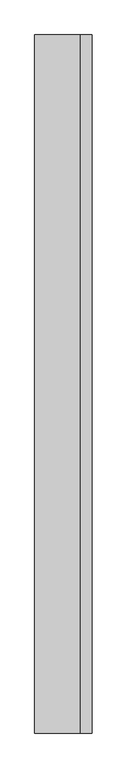
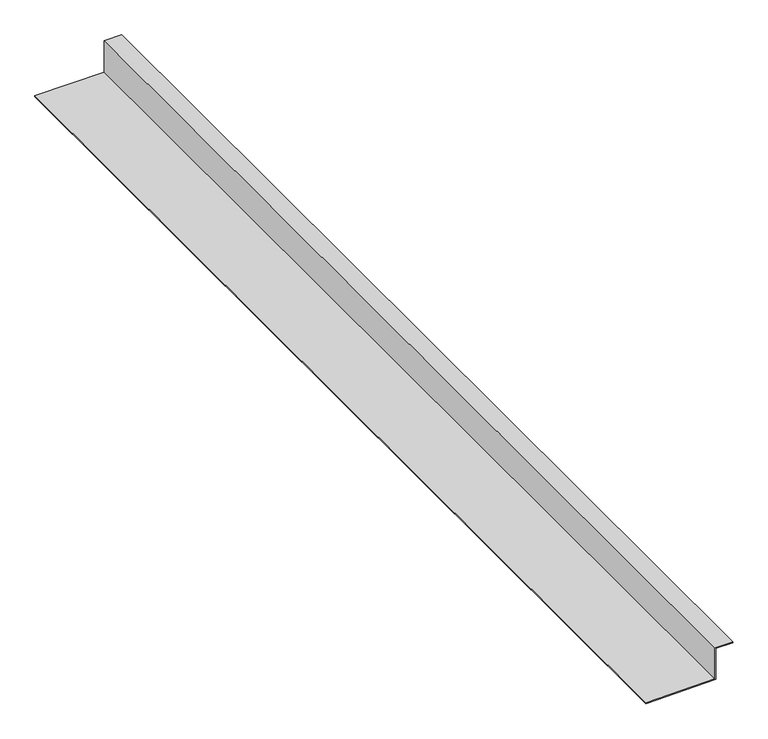
"""IFC4 building model written with IfcOpenShell, lengths in millimetres: proxy geometry, Membrane058 4483 : Membrane058 4483."""

from ifc_helpers import new_model, si_unit, frame, origin, place, context, project, spatial, polyline, outline, extrude, source, transform, mapped, element, save


def generic_models_554ca42b(model_context):
    return source(origin(), model_context, "Body", "SweptSolid", [
        extrude(outline(polyline([(40320.2734375, -1061.1228027), (40320.2734375, -1094.7133789), (40257.7779451, -1094.7133789), (40256.0193501, -1225.3491868), (40254.0195312, -1225.3222656), (40255.8046875, -1092.7133789), (40318.2734375, -1092.7133789), (40318.2734375, -1061.1228027), (40320.2734375, -1061.1228027)])), frame((0.0, -1052.8906574, 0.0), z_axis=(0.0, 1.0, 0.0), x_axis=(0.0, 0.0, 1.0)), (0.0, 0.0, 1.0), 2000.0),
    ])


if __name__ == "__main__":
    model = new_model("IFC4")
    model_context = context("Model", 3, world=origin())
    ifc_project = project(units=[si_unit("LENGTHUNIT", "METRE", prefix="MILLI")], contexts=[model_context])
    site = spatial("IfcSite", under=ifc_project)
    building = spatial("IfcBuilding", under=site)
    placement = place(None, origin())
    generic_models_shape = generic_models_554ca42b(model_context)
    element("IfcBuildingElementProxy", 1, Name="Membrane058 4483 : Membrane058 4483", ObjectType="Membrane058 4483 : Membrane058 4483", at=placement, inside=building, context=model_context, shape_type="MappedRepresentation", body=[
        mapped(generic_models_shape, transform((0.0, 0.0, 0.0), x_axis=(1.0, 0.0, 0.0), y_axis=(0.0, 1.0, 0.0), z_axis=(0.0, 0.0, 1.0))),
    ])
    save(model, "model.ifc")

# Revit data of these elements
# Type "Membrane058 4483 : Membrane058 4483"
#   NameOverride = "Membrane058"
# Element 1 (IfcBuildingElementProxy, "Membrane058 4483 : Membrane058 4483")
#   Materials on its faces: "BITUMINOUS BUILT-UP ROOF MEMBRANE"
# Materials
#   "BITUMINOUS BUILT-UP ROOF MEMBRANE": class "Unassigned", colour RGB 34 145 0, transparency 0
